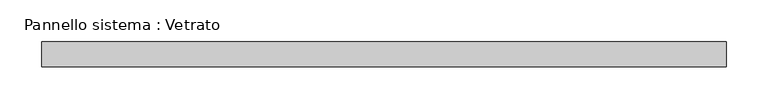
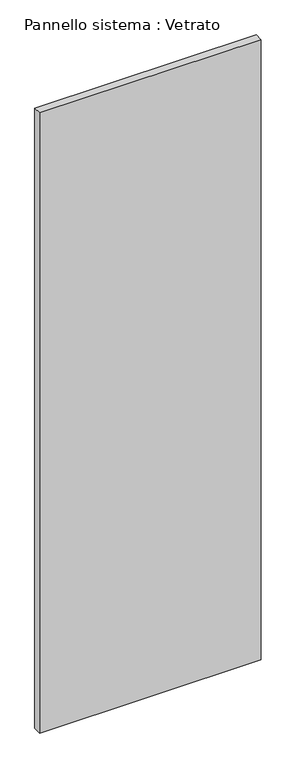
"""IFC4 building model written with IfcOpenShell, lengths in millimetres: plate geometry, Pannello sistema : Vetrato."""

from ifc_helpers import new_model, si_unit, origin, origin_with_axes, place, context, project, spatial, polyline, outline, extrude, source, transform, mapped, element, save


def pannello_sistema_vetrato_2bfc7cdc(model_context):
    return source(origin(), model_context, "Body", "SweptSolid", [
        extrude(outline(polyline([(410.0, -15.0), (-410.0, -15.0), (-410.0, 15.0), (410.0, 15.0), (410.0, -15.0)])), origin_with_axes(), (0.0, 0.0, 1.0), 2425.0),
    ])


if __name__ == "__main__":
    model = new_model("IFC4")
    model_context = context("Model", 3, world=origin())
    ifc_project = project(units=[si_unit("LENGTHUNIT", "METRE", prefix="MILLI")], contexts=[model_context])
    site = spatial("IfcSite", under=ifc_project)
    building = spatial("IfcBuilding", under=site)
    placement = place(None, origin())
    pannello_sistema_vetrato_shape = pannello_sistema_vetrato_2bfc7cdc(model_context)
    element("IfcPlate", 1, ObjectType="Pannello sistema : Vetrato", at=placement, inside=building, context=model_context, shape_type="MappedRepresentation", body=[
        mapped(pannello_sistema_vetrato_shape, transform((0.0, 0.0, 0.0), x_axis=(1.0, 0.0, 0.0), y_axis=(0.0, 1.0, 0.0), z_axis=(0.0, 0.0, 1.0))),
    ])
    save(model, "model.ifc")

# Revit data of these elements
# Type "Pannello sistema : Vetrato"
#   Construction Type Id = "GSP4R"
#   Analytic Construction = "Vetrata singola Pilkington 1/8 in"
#   Visual Light Transmittance = 0.9
#   Solar Heat Gain Coefficient = 0.86
#   Heat Transfer Coefficient (U) = 6.7069 W/(m²·K)
# Element 1 (IfcPlate, "Pannello sistema : Vetrato")
#   Materials on its faces: "Default - Vetro"
# Materials
#   "Default - Vetro": class "Vetro", colour RGB 208 208 208, transparency 0.7, Cost = 0
